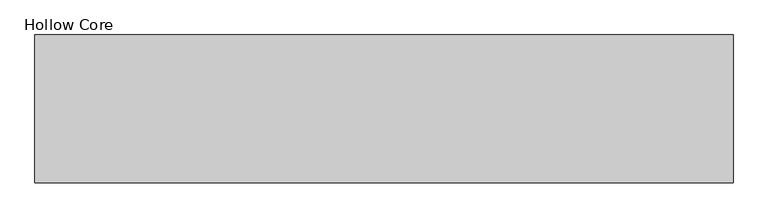
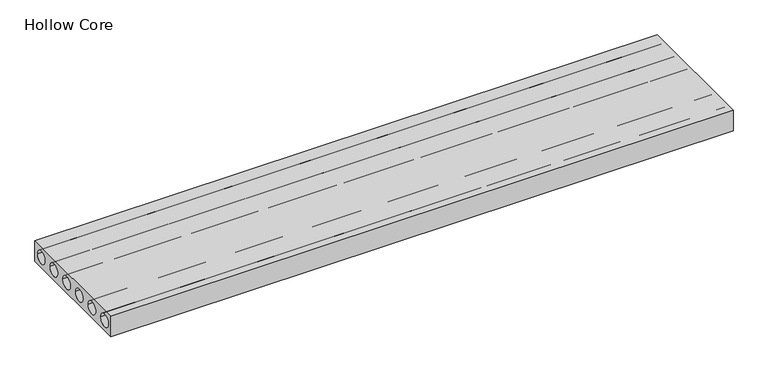
"""IFC4 building model written with IfcOpenShell, lengths in millimetres: proxy geometry, Hollow Core : Breton Hollow Core."""

from ifc_helpers import new_model, si_unit, point, frame, frame_2d, origin, place, context, project, spatial, polyline, circle_curve, trimmed, segment, composite_curve, outline, extrude, source, transform, mapped, element, save


def hollow_core_b1c9e8cf(model_context):
    return source(origin(), model_context, "Body", "SweptSolid", [
        extrude(outline(polyline([(-609.6, 100.0), (609.6, 100.0), (609.6, -100.0), (-609.6, -100.0), (-609.6, 100.0)]), holes=[composite_curve([segment(trimmed(circle_curve(frame_2d((508.0, 0.0)), 60.0), [point((448.0, 0.0))], [point((568.0, 0.0))], True, "CARTESIAN"), True, "CONTINUOUS"), segment(trimmed(circle_curve(frame_2d((508.0, 0.0)), 60.0), [point((568.0, 0.0))], [point((448.0, 0.0))], True, "CARTESIAN"), True, "CONTINUOUS")], self_intersect=False), composite_curve([segment(trimmed(circle_curve(frame_2d((-508.0, 0.0)), 60.0), [point((-568.0, 0.0))], [point((-448.0, 0.0))], True, "CARTESIAN"), True, "CONTINUOUS"), segment(trimmed(circle_curve(frame_2d((-508.0, 0.0)), 60.0), [point((-448.0, 0.0))], [point((-568.0, 0.0))], True, "CARTESIAN"), True, "CONTINUOUS")], self_intersect=False), composite_curve([segment(trimmed(circle_curve(frame_2d((304.8, 0.0)), 60.0), [point((244.8, 0.0))], [point((364.8, 0.0))], True, "CARTESIAN"), True, "CONTINUOUS"), segment(trimmed(circle_curve(frame_2d((304.8, 0.0)), 60.0), [point((364.8, 0.0))], [point((244.8, 0.0))], True, "CARTESIAN"), True, "CONTINUOUS")], self_intersect=False), composite_curve([segment(trimmed(circle_curve(frame_2d((101.6, 0.0)), 60.0), [point((41.6, 0.0))], [point((161.6, 0.0))], True, "CARTESIAN"), True, "CONTINUOUS"), segment(trimmed(circle_curve(frame_2d((101.6, 0.0)), 60.0), [point((161.6, 0.0))], [point((41.6, 0.0))], True, "CARTESIAN"), True, "CONTINUOUS")], self_intersect=False), composite_curve([segment(trimmed(circle_curve(frame_2d((-101.6, 0.0)), 60.0), [point((-161.6, 0.0))], [point((-41.6, 0.0))], True, "CARTESIAN"), True, "CONTINUOUS"), segment(trimmed(circle_curve(frame_2d((-101.6, 0.0)), 60.0), [point((-41.6, 0.0))], [point((-161.6, 0.0))], True, "CARTESIAN"), True, "CONTINUOUS")], self_intersect=False), composite_curve([segment(trimmed(circle_curve(frame_2d((-304.8, 0.0)), 60.0), [point((-364.8, 0.0))], [point((-244.8, 0.0))], True, "CARTESIAN"), True, "CONTINUOUS"), segment(trimmed(circle_curve(frame_2d((-304.8, 0.0)), 60.0), [point((-244.8, 0.0))], [point((-364.8, 0.0))], True, "CARTESIAN"), True, "CONTINUOUS")], self_intersect=False)]), frame((0.0, 0.0, 0.0), z_axis=(1.0, 0.0, 0.0), x_axis=(0.0, 1.0, 0.0)), (0.0, 0.0, 1.0), 5760.0),
    ])


if __name__ == "__main__":
    model = new_model("IFC4")
    model_context = context("Model", 3, world=origin())
    ifc_project = project(units=[si_unit("LENGTHUNIT", "METRE", prefix="MILLI")], contexts=[model_context])
    site = spatial("IfcSite", under=ifc_project)
    building = spatial("IfcBuilding", under=site)
    placement = place(None, origin())
    hollow_core_shape = hollow_core_b1c9e8cf(model_context)
    element("IfcBuildingElementProxy", 1, Name="Hollow Core : Breton Hollow Core", ObjectType="Hollow Core : Breton Hollow Core", at=placement, inside=building, context=model_context, shape_type="MappedRepresentation", body=[
        mapped(hollow_core_shape, transform((0.0, 0.0, 0.0), x_axis=(1.0, 0.0, 0.0), y_axis=(0.0, 1.0, 0.0), z_axis=(0.0, 0.0, 1.0))),
    ])
    save(model, "model.ifc")

# Revit data of these elements
# Type "Hollow Core : Breton Hollow Core"
#   Width [instance default] = 1219.2 mm
#   built-in parameter 1001306 [instance default] = 4 (stored number, unit not read)
#   Depth [instance default] = 152.4 mm
#   Core Radius [instance default] = 50.8 mm
#   Core Offset [instance default] = 101.6 mm
#   Number Of Cores [instance default] = 2
#   Material [instance default] = Concrete - Precast Concrete - Normal Weight - 5 ksi
#   Default Elevation = 0
#   Assembly Code = ""
# Element 1 (IfcBuildingElementProxy, "Hollow Core : Breton Hollow Core")
#   built-in parameter 1001306 = 18.8976 (stored number, unit not read)
#   Depth = 200 mm
#   Core Radius = 60 mm
#   Number Of Cores = 6
#   Materials on its faces: "Concrete - Precast Concrete - Normal Weight - 5 ksi"
# Materials
#   "Concrete - Precast Concrete - Normal Weight - 5 ksi": class "Concrete", colour RGB 198 187 187, transparency 0
